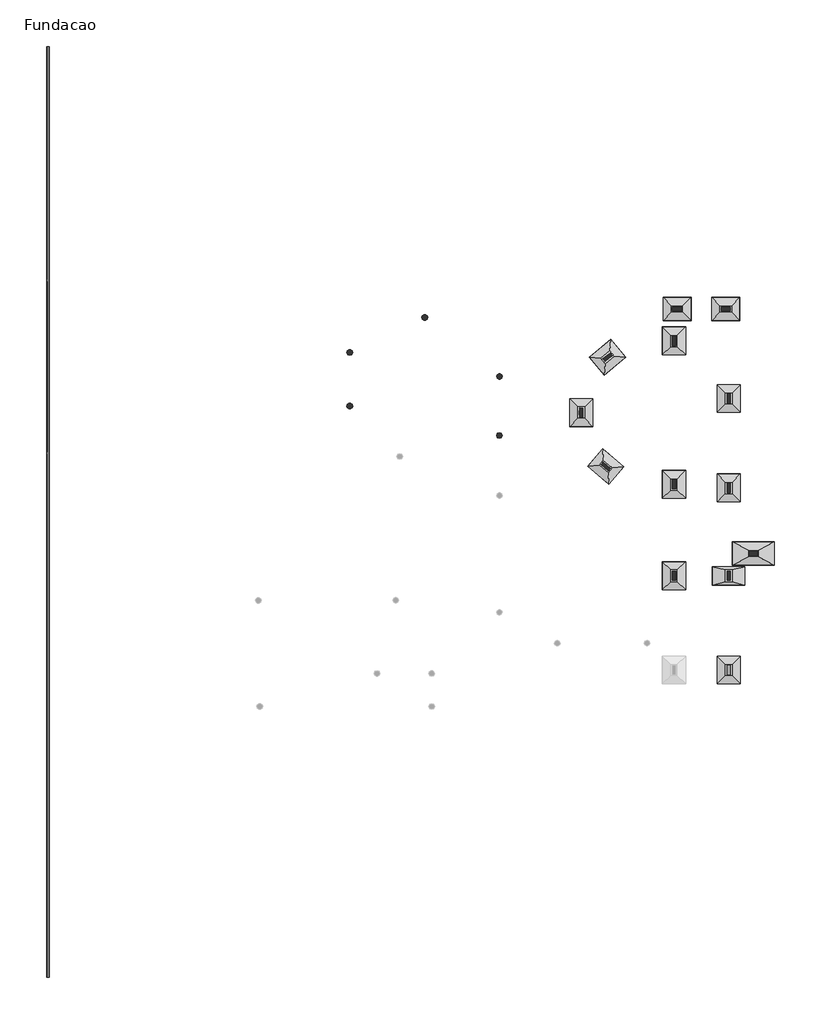
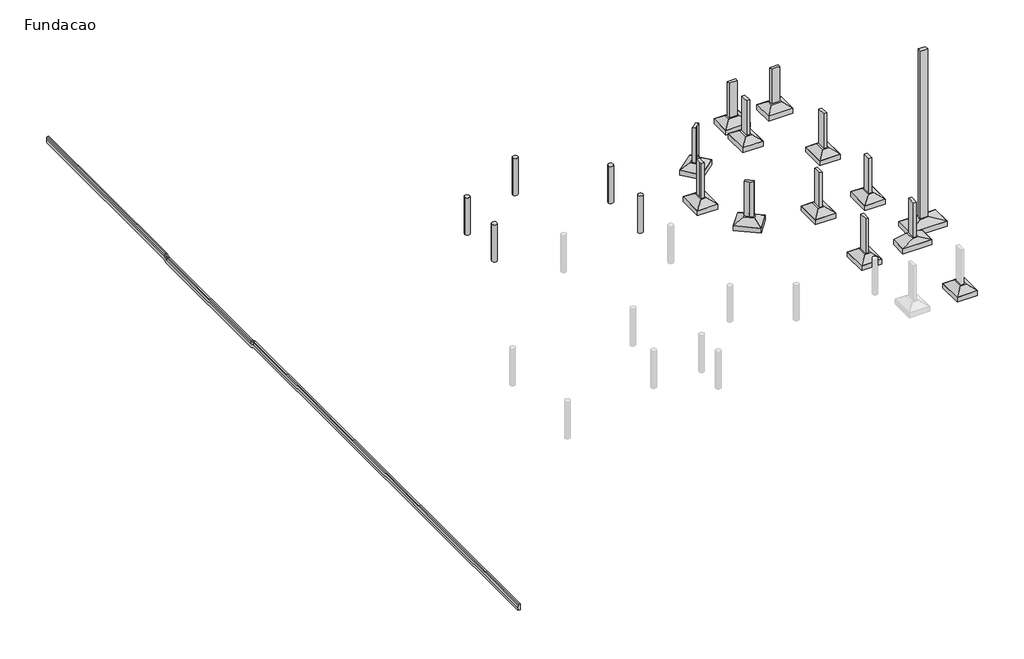
# One storey, part 2 of 2: 17 columns, 13 fasteners, 1 proxy.
"""IFC4 building model written with IfcOpenShell, lengths in millimetres."""

import ifcopenshell
import ifcopenshell.guid

model = None  # the IFC model being written
_history = None  # IfcOwnerHistory: only IFC2X3 demands one
_inside = {}  # id of a spatial element -> (the spatial element, [elements in it])
_under = {}  # id of a project, library or spatial element -> (it, [spatial elements below it])
_declared = {}  # id of a project -> (the project, [libraries it declares])
_typed = {}  # id of a type object -> (the type object, [elements of that type])
_made_of = {}  # id of a material, layer set ... -> (it, [elements and type objects made of it])


def new_model(schema):
    """Start an empty IFC model of exactly this schema.

    Asked for "IFC4X3", IfcOpenShell would pick the latest addendum, in which some entities
    have other attributes; the version numbers below select the first issue.
    IFC2X3 requires an IfcOwnerHistory on every rooted entity: one is made here for all.
    """
    global model, _history
    if schema == "IFC4X3":
        model = ifcopenshell.file(schema_version=(4, 3, 0, 0))
    else:
        model = ifcopenshell.file(schema=schema)
    _inside.clear()
    _under.clear()
    _declared.clear()
    _typed.clear()
    _made_of.clear()
    _history = None
    if model.schema == "IFC2X3":
        org = make("IfcOrganization", Name="unknown")
        user = make(
            "IfcPersonAndOrganization",
            ThePerson=make("IfcPerson", FamilyName="unknown"),
            TheOrganization=org,
        )
        app = make(
            "IfcApplication",
            ApplicationDeveloper=org,
            Version="unknown",
            ApplicationFullName="unknown",
            ApplicationIdentifier="unknown",
        )
        _history = make(
            "IfcOwnerHistory",
            OwningUser=user,
            OwningApplication=app,
            ChangeAction="ADDED",
            CreationDate=0,
        )
    return model


def make(cls, **values):
    """One entity of the class cls with the attributes given. An attribute that is None is left unset."""
    return model.create_entity(
        cls, **{name: value for name, value in values.items() if value is not None}
    )


def rooted(cls, **values):
    """An entity with a GlobalId (a new one), such as an element, a storey or a relation."""
    return make(cls, GlobalId=ifcopenshell.guid.new(), OwnerHistory=_history, **values)


def si_unit(unit_type, name, prefix=None):
    """IfcSIUnit, for example si_unit("LENGTHUNIT", "METRE", prefix="MILLI")."""
    return make("IfcSIUnit", UnitType=unit_type, Prefix=prefix, Name=name)


def assignment(units):
    """IfcUnitAssignment: the units of a project."""
    return None if units is None else make("IfcUnitAssignment", Units=units)


def point(xyz):
    """IfcCartesianPoint."""
    return None if xyz is None else make("IfcCartesianPoint", Coordinates=xyz)


def direction(xyz):
    """IfcDirection."""
    return None if xyz is None else make("IfcDirection", DirectionRatios=xyz)


def frame(location, z_axis=None, x_axis=None):
    """IfcAxis2Placement3D, a coordinate frame: its origin and axes. An axis left out is left unset."""
    return make(
        "IfcAxis2Placement3D",
        Location=point(location),
        Axis=direction(z_axis),
        RefDirection=direction(x_axis),
    )


def origin():
    """The frame at (0, 0, 0) with its axes left unset."""
    return frame((0.0, 0.0, 0.0))


def place(relative_to, where):
    """IfcLocalPlacement: puts the frame where relative to a parent placement (None: the world)."""
    return make(
        "IfcLocalPlacement", PlacementRelTo=relative_to, RelativePlacement=where
    )


def context(
    kind, dimensions, precision=None, world=None, true_north=None, identifier=None
):
    """IfcGeometricRepresentationContext, for example the 3D "Model" context."""
    return make(
        "IfcGeometricRepresentationContext",
        ContextIdentifier=identifier,
        ContextType=kind,
        CoordinateSpaceDimension=dimensions,
        Precision=precision,
        WorldCoordinateSystem=world,
        TrueNorth=true_north,
    )


def project(units=None, contexts=None):
    """IfcProject with its units and contexts."""
    return rooted(
        "IfcProject",
        Name="project",
        RepresentationContexts=contexts,
        UnitsInContext=assignment(units),
    )


def spatial(cls, under=None, at=None, **own):
    """A site, building, storey or space (cls), placed at a placement, below another one or the project."""
    s = rooted(cls, ObjectPlacement=at, **own)
    if under is not None:
        _under.setdefault(under.id(), (under, []))[1].append(s)
    return s


def polyline(points):
    """IfcPolyline through the points."""
    return make("IfcPolyline", Points=[point(p) for p in points])


def circle_curve(where, radius):
    """IfcCircle in the frame where."""
    return make("IfcCircle", Position=where, Radius=radius)


def ellipse_curve(where, semi_axis1, semi_axis2):
    """IfcEllipse in the frame where."""
    return make(
        "IfcEllipse", Position=where, SemiAxis1=semi_axis1, SemiAxis2=semi_axis2
    )


def outline(outer, holes=None, kind="AREA"):
    """IfcArbitraryClosedProfileDef: a profile drawn as a closed curve; with holes, ...WithVoids."""
    if holes is None:
        return make("IfcArbitraryClosedProfileDef", ProfileType=kind, OuterCurve=outer)
    return make(
        "IfcArbitraryProfileDefWithVoids",
        ProfileType=kind,
        OuterCurve=outer,
        InnerCurves=holes,
    )


def extrude(swept, where, along, depth):
    """IfcExtrudedAreaSolid: the profile swept, set in the frame where, extruded along a direction by depth."""
    return make(
        "IfcExtrudedAreaSolid",
        SweptArea=swept,
        Position=where,
        ExtrudedDirection=direction(along),
        Depth=depth,
    )


def faces_of(points, faces, orient=None, outer=None):
    """IfcFace entities. A face is a list of loops; a loop is a list of indices into points, from 0.

    orient and outer hold one flag for each loop. By default every Orientation is true, the
    first loop of a face is its IfcFaceOuterBound and the others are IfcFaceBound.
    """
    made = []
    for i, loops in enumerate(faces):
        bounds = []
        for j, loop in enumerate(loops):
            is_outer = j == 0 if outer is None else outer[i][j]
            bounds.append(
                make(
                    "IfcFaceOuterBound" if is_outer else "IfcFaceBound",
                    Bound=make("IfcPolyLoop", Polygon=[points[k] for k in loop]),
                    Orientation=True if orient is None else orient[i][j],
                )
            )
        made.append(make("IfcFace", Bounds=bounds))
    return made


def faceted_brep(points, faces, orient=None, outer=None, voids=None):
    """IfcFacetedBrep: a solid bounded by flat faces; with voids (closed shells), ...WithVoids."""
    shared = [point(p) for p in points]
    hull = make("IfcClosedShell", CfsFaces=faces_of(shared, faces, orient, outer))
    if voids is None:
        return make("IfcFacetedBrep", Outer=hull)
    return make(
        "IfcFacetedBrepWithVoids",
        Outer=hull,
        Voids=[
            make(cls, CfsFaces=faces_of(shared, fs, o, b)) for cls, fs, o, b in voids
        ],
    )


def shape(context_of_items, identifier, shape_type, items):
    """IfcShapeRepresentation: the items that make up one representation, for example the "Body"."""
    return make(
        "IfcShapeRepresentation",
        ContextOfItems=context_of_items,
        RepresentationIdentifier=identifier,
        RepresentationType=shape_type,
        Items=items,
    )


def source(mapping_origin, context_of_items, identifier, shape_type, items):
    """IfcRepresentationMap: a shape defined once, which mapped items show again and again."""
    return make(
        "IfcRepresentationMap",
        MappingOrigin=mapping_origin,
        MappedRepresentation=shape(context_of_items, identifier, shape_type, items),
    )


def transform(
    local_origin,
    x_axis=None,
    y_axis=None,
    z_axis=None,
    scale=None,
    scale2=None,
    scale3=None,
    uniform=True,
):
    """IfcCartesianTransformationOperator3D, or its non-uniform kind. x_axis, y_axis, z_axis: its Axis1, 2, 3."""
    if uniform:
        return make(
            "IfcCartesianTransformationOperator3D",
            Axis1=direction(x_axis),
            Axis2=direction(y_axis),
            LocalOrigin=point(local_origin),
            Scale=scale,
            Axis3=direction(z_axis),
        )
    return make(
        "IfcCartesianTransformationOperator3DnonUniform",
        Axis1=direction(x_axis),
        Axis2=direction(y_axis),
        LocalOrigin=point(local_origin),
        Scale=scale,
        Axis3=direction(z_axis),
        Scale2=scale2,
        Scale3=scale3,
    )


def mapped(mapping_source, mapping_target):
    """IfcMappedItem: shows the shape of a source again, moved by a transform."""
    return make(
        "IfcMappedItem", MappingSource=mapping_source, MappingTarget=mapping_target
    )


def made_of(thing, what):
    """Note that an element or type object is made of a material, layer set ...; save() writes the relation."""
    if what is not None:
        _made_of.setdefault(what.id(), (what, []))[1].append(thing)
    return thing


def element(
    cls,
    number,
    at=None,
    inside=None,
    cuts=None,
    type_object=None,
    material=None,
    context=None,
    identifier="Body",
    shape_type=None,
    held_by="IfcProductDefinitionShape",
    body=None,
    shapes=None,
    **own,
):
    """One element of the class cls, such as IfcWall. Its Tag is "e" and its number.

    at: its placement. inside: the storey or other place that contains it. cuts: it is an
    opening in that element (IfcRelVoidsElement). A single representation is given by context,
    identifier, shape_type and body (its items); several are given by shapes. held_by: the class
    of the entity that holds the representations. save() writes the other relations.
    """
    e = rooted(cls, Tag="e%d" % number, ObjectPlacement=at, **own)
    if body is not None:
        shapes = [shape(context, identifier, shape_type, body)]
    if shapes is not None:
        e.Representation = make(held_by, Representations=shapes)
    if inside is not None:
        _inside.setdefault(inside.id(), (inside, []))[1].append(e)
    if cuts is not None:
        rooted(
            "IfcRelVoidsElement", RelatingBuildingElement=cuts, RelatedOpeningElement=e
        )
    if type_object is not None:
        _typed.setdefault(type_object.id(), (type_object, []))[1].append(e)
    return made_of(e, material)


def aggregate(whole, parts):
    """IfcRelAggregates: a whole, such as a stair, and the parts it consists of."""
    return rooted("IfcRelAggregates", RelatingObject=whole, RelatedObjects=parts)


def save(model, path):
    """Write the relations noted so far, then the file.

    IfcRelAggregates (storeys below a building ...), IfcRelContainedInSpatialStructure (elements
    in a storey), IfcRelDefinesByType, IfcRelAssociatesMaterial and IfcRelDeclares: one each for
    every whole, place, type object, material and project.
    """
    for whole, parts in _under.values():
        aggregate(whole, parts)
    for where, things in _inside.values():
        rooted(
            "IfcRelContainedInSpatialStructure",
            RelatedElements=things,
            RelatingStructure=where,
        )
    for kind, things in _typed.values():
        rooted("IfcRelDefinesByType", RelatedObjects=things, RelatingType=kind)
    for what, things in _made_of.values():
        rooted("IfcRelAssociatesMaterial", RelatedObjects=things, RelatingMaterial=what)
    for by, libraries in _declared.values():
        rooted("IfcRelDeclares", RelatingContext=by, RelatedDefinitions=libraries)
    model.write(path)


def plane_surface(at):
    """IfcPlane: the flat surface through the origin of the frame at, square to its z axis."""
    return make("IfcPlane", Position=at)


def cylinder_surface(at, radius):
    """IfcCylindricalSurface: all points at the distance radius from the z axis of the frame at."""
    return make("IfcCylindricalSurface", Position=at, Radius=radius)


def advanced_brep(points, edges, surfaces, faces):
    """IfcAdvancedBrep: a solid bounded by faces that lie on surfaces and meet in shared edges.

    An edge is (start, end): straight between two places in points (the first is 0);
    or (start, end, curve); or (start, end, curve, False) where it runs against its curve.
    A face is (place in surfaces, loops), or (place, loops, False) where it looks against
    its surface's normal. A loop lists edges by number (the first is 1), with a minus sign
    where the edge is run from its end to its start. The first loop is the outer one.
    """
    corners = [point(p) for p in points]
    vertices = [make("IfcVertexPoint", VertexGeometry=c) for c in corners]
    made = []
    for start, end, *more in edges:
        made.append(
            make(
                "IfcEdgeCurve",
                EdgeStart=vertices[start],
                EdgeEnd=vertices[end],
                EdgeGeometry=more[0] if more else make("IfcPolyline", Points=[corners[start], corners[end]]),
                SameSense=more[1] if len(more) > 1 else True,
            )
        )
    hull = []
    for where, loops, *sense in faces:
        bounds = []
        for j, loop in enumerate(loops):
            ring = [make("IfcOrientedEdge", EdgeElement=made[abs(k) - 1], Orientation=k > 0) for k in loop]
            bounds.append(
                make(
                    "IfcFaceOuterBound" if j == 0 else "IfcFaceBound",
                    Bound=make("IfcEdgeLoop", EdgeList=ring),
                    Orientation=True,
                )
            )
        hull.append(make("IfcAdvancedFace", Bounds=bounds, FaceSurface=surfaces[where], SameSense=sense[0] if sense else True))
    return make("IfcAdvancedBrep", Outer=make("IfcClosedShell", CfsFaces=hull))


def meio_fio_meio_fio_c5939b1e(model_context):
    return source(origin(), model_context, "Body", "AdvancedBrep", [
        advanced_brep(
        [(-19460.281307, 17327.5225294, 100.0), (-19460.281307, 17327.5225294, -200.0), (-19580.281307, 17327.5225294, -200.0), (-19580.281307, 17327.5225294, -50.0), (-19560.334366, 17327.5225294, 74.7371665), (-19530.7107394, 17327.5225294, 100.0), (-19460.281307, 7304.4300153, 100.0), (-19460.281307, 7104.4300153, 20.0), (-19460.281307, 4.4300153, 20.0), (-19460.281307, -195.5699847, 100.0), (-19460.281307, -22700.938406, 100.0), (-19460.281307, -22700.938406, -200.0), (-19460.281307, -253.3447058, -200.0), (-19460.281307, -53.3447058, -280.0), (-19460.281307, 7162.2047364, -280.0), (-19460.281307, 7362.2047364, -200.0), (-19580.281307, 7362.2047364, -200.0), (-19580.281307, 7162.2047364, -280.0), (-19580.281307, -53.3447058, -280.0), (-19580.281307, -253.3447058, -200.0), (-19580.281307, -22700.938406, -200.0), (-19580.281307, -22700.938406, -50.0), (-19580.281307, -224.4573452, -50.0), (-19580.281307, -24.4573452, -130.0), (-19580.281307, 7133.3173758, -130.0), (-19580.281307, 7333.3173758, -50.0), (-19560.334366, 7309.2951925, 74.7371665), (-19530.7107394, 7304.4300153, 100.0), (-19560.334366, 7109.2951925, -5.2628335), (-19530.7107394, 7104.4300153, 20.0), (-19560.334366, -0.4351619, -5.2628335), (-19530.7107394, 4.4300153, 20.0), (-19560.334366, -200.4351619, 74.7371665), (-19530.7107394, -195.5699847, 100.0), (-19530.7107394, -22700.938406, 100.0), (-19560.334366, -22700.938406, 74.7371665)],
        [
            (0, 1),
            (1, 2),
            (2, 3),
            (3, 4),
            (4, 5, circle_curve(frame((-19530.7107394, 17327.5225294, 70.0), z_axis=(0.0, 1.0, 0.0), x_axis=(-1.0, 0.0, 0.0)), 30.0)),
            (5, 0),
            (0, 6),
            (6, 7),
            (7, 8),
            (8, 9),
            (9, 10),
            (10, 11),
            (11, 12),
            (12, 13),
            (13, 14),
            (14, 15),
            (15, 1),
            (15, 16),
            (16, 2),
            (16, 17),
            (17, 18),
            (18, 19),
            (19, 20),
            (20, 21),
            (21, 22),
            (22, 23),
            (23, 24),
            (24, 25),
            (25, 3),
            (25, 26),
            (26, 4),
            (26, 27, ellipse_curve(frame((-19530.7107394, 7310.2074874, 70.0), z_axis=(0.0, 0.9819563867314226, 0.18910752115494767), x_axis=(0.0, 0.18910752115494667, -0.9819563867314226)), 30.551255, 30.0)),
            (27, 5),
            (27, 6),
            (14, 17),
            (24, 28),
            (28, 26),
            (28, 29, ellipse_curve(frame((-19530.7107394, 7110.2074874, -10.0), z_axis=(0.0, 0.9819563867314226, 0.18910752115494764), x_axis=(0.0, -0.18910752115494842, 0.9819563867314223)), 30.551255, 30.0)),
            (29, 27),
            (29, 7),
            (13, 18),
            (23, 30),
            (30, 28),
            (30, 31, ellipse_curve(frame((-19530.7107394, -1.3474568, -10.0), z_axis=(0.0, 0.9819563867314217, -0.1891075211549513), x_axis=(0.0, 0.18910752115495252, 0.9819563867314217)), 30.551255, 30.0)),
            (31, 29),
            (31, 8),
            (12, 19),
            (22, 32),
            (32, 30),
            (32, 33, ellipse_curve(frame((-19530.7107394, -201.3474568, 70.0), z_axis=(0.0, 0.9819563867314217, -0.18910752115495139), x_axis=(0.0, -0.18910752115495078, -0.9819563867314218)), 30.551255, 30.0)),
            (33, 31),
            (33, 9),
            (10, 34),
            (34, 35, circle_curve(frame((-19530.7107394, -22700.938406, 70.0), z_axis=(0.0, -1.0, 0.0), x_axis=(-1.0, 0.0, 0.0)), 30.0)),
            (35, 21),
            (20, 11),
            (35, 32),
            (34, 33),
        ],
        [
            plane_surface(frame((-19460.281307, 17327.5225294, 100.0), z_axis=(0.0, 1.0, 0.0), x_axis=(0.0, 0.0, 1.0))),
            plane_surface(frame((-19460.281307, 17327.5225294, 100.0), z_axis=(1.0, 0.0, 0.0), x_axis=(0.0, -1.0, 0.0))),
            plane_surface(frame((-19460.281307, 17327.5225294, -200.0), z_axis=(0.0, 0.0, -1.0), x_axis=(0.0, -1.0, 0.0))),
            plane_surface(frame((-19580.281307, 17327.5225294, -200.0), z_axis=(-1.0, 0.0, 0.0), x_axis=(0.0, -1.0, 0.0))),
            plane_surface(frame((-19580.281307, 17327.5225294, -50.0), z_axis=(-0.9874542202157147, 0.0, 0.15790555081495689), x_axis=(0.0, -1.0, 0.0))),
            cylinder_surface(frame((-19530.7107394, 17327.5225294, 70.0), z_axis=(0.0, 1.0, 0.0), x_axis=(-1.0, 0.0, 0.0)), 30.0),
            plane_surface(frame((-19530.7107394, 17327.5225294, 100.0), z_axis=(0.0, 0.0, 1.0), x_axis=(0.0, -1.0, 0.0))),
            plane_surface(frame((-19460.281307, 7362.2047364, -200.0), z_axis=(0.0, 0.3713906763540969, -0.9284766908852621), x_axis=(0.0, -0.9284766908852621, -0.3713906763540969))),
            plane_surface(frame((-19580.281307, 7333.3173758, -50.0), z_axis=(-0.9874542202157147, -0.05864464931723302, 0.1466116232930858), x_axis=(0.0, -0.9284766908852622, -0.3713906763540966))),
            cylinder_surface(frame((-19530.7107394, 7315.5717356, 72.1456993), z_axis=(0.0, 0.9284766908852621, 0.3713906763540969), x_axis=(-1.0, 0.0, 0.0)), 30.0),
            plane_surface(frame((-19530.7107394, 7304.4300153, 100.0), z_axis=(0.0, -0.37139067635409667, 0.9284766908852622), x_axis=(0.0, -0.9284766908852622, -0.37139067635409667))),
            plane_surface(frame((-19460.281307, 7162.2047364, -280.0), z_axis=(0.0, 0.0, -1.0), x_axis=(0.0, -1.0, 0.0))),
            plane_surface(frame((-19580.281307, 7133.3173758, -130.0), z_axis=(-0.9874542202157146, 0.0, 0.15790555081495686), x_axis=(0.0, -1.0, 0.0))),
            cylinder_surface(frame((-19530.7107394, 7104.4300153, -10.0), z_axis=(0.0, 1.0, 0.0), x_axis=(-1.0, 0.0, 0.0)), 30.0),
            plane_surface(frame((-19530.7107394, 7104.4300153, 20.0), z_axis=(0.0, 0.0, 1.0), x_axis=(0.0, -1.0, 0.0))),
            plane_surface(frame((-19460.281307, -53.3447058, -280.0), z_axis=(0.0, -0.37139067635410367, -0.9284766908852594), x_axis=(0.0, -0.9284766908852594, 0.37139067635410367))),
            plane_surface(frame((-19580.281307, -24.4573452, -130.0), z_axis=(-0.9874542202157147, 0.05864464931723411, 0.14661162329308536), x_axis=(0.0, -0.9284766908852594, 0.37139067635410355))),
            cylinder_surface(frame((-19530.7107394, -6.711705, -7.8543007), z_axis=(0.0, 0.9284766908852593, -0.3713906763541038), x_axis=(-1.0, 0.0, 0.0)), 30.0),
            plane_surface(frame((-19530.7107394, 4.4300153, 20.0), z_axis=(0.0, 0.3713906763541038, 0.9284766908852593), x_axis=(0.0, -0.9284766908852593, 0.3713906763541038))),
            plane_surface(frame((-19460.281307, -22700.938406, 100.0), z_axis=(0.0, -1.0, 0.0), x_axis=(0.0, 0.0, 1.0))),
            plane_surface(frame((-19460.281307, -253.3447058, -200.0), z_axis=(0.0, 0.0, -1.0), x_axis=(0.0, -1.0, 0.0))),
            plane_surface(frame((-19580.281307, -224.4573452, -50.0), z_axis=(-0.9874542202157146, 0.0, 0.15790555081495683), x_axis=(0.0, -1.0, 0.0))),
            cylinder_surface(frame((-19530.7107394, -195.5699847, 70.0), z_axis=(0.0, 1.0, 0.0), x_axis=(-1.0, 0.0, 0.0)), 30.0),
            plane_surface(frame((-19530.7107394, -195.5699847, 100.0), z_axis=(0.0, 0.0, 1.0), x_axis=(0.0, -1.0, 0.0))),
        ],
        [
            (0, [[1, 2, 3, 4, 5, 6]]),
            (1, [[-1, 7, 8, 9, 10, 11, 12, 13, 14, 15, 16, 17]]),
            (2, [[-2, -17, 18, 19]]),
            (3, [[-3, -19, 20, 21, 22, 23, 24, 25, 26, 27, 28, 29]]),
            (4, [[-4, -29, 30, 31]]),
            (5, [[-5, -31, 32, 33]]),
            (6, [[-6, -33, 34, -7]]),
            (7, [[-18, -16, 35, -20]]),
            (8, [[-30, -28, 36, 37]]),
            (9, [[-32, -37, 38, 39]]),
            (10, [[-34, -39, 40, -8]]),
            (11, [[-35, -15, 41, -21]]),
            (12, [[-36, -27, 42, 43]]),
            (13, [[-38, -43, 44, 45]]),
            (14, [[-40, -45, 46, -9]]),
            (15, [[-41, -14, 47, -22]]),
            (16, [[-42, -26, 48, 49]]),
            (17, [[-44, -49, 50, 51]]),
            (18, [[-46, -51, 52, -10]]),
            (19, [[53, 54, 55, -24, 56, -12]]),
            (20, [[-47, -13, -56, -23]]),
            (21, [[-48, -25, -55, 57]]),
            (22, [[-50, -57, -54, 58]]),
            (23, [[-52, -58, -53, -11]]),
        ],
    ),
    ])


def s14_8166d2be(model_context):
    return source(origin(), model_context, "Body", "SolidModel", [
        faceted_brep([(-55.0, 0.0, 0.0), (-345.0, 0.0, 0.0), (-345.0, -400.0, 0.0), (-55.0, -400.0, 0.0), (300.0, 700.0, -250.0), (300.0, -1100.0, -250.0), (-700.0, -1100.0, -250.0), (-700.0, 700.0, -250.0)], [[[0, 1, 2, 3]], [[4, 5, 6, 7]], [[4, 7, 1, 0]], [[7, 6, 2, 1]], [[6, 5, 3, 2]], [[5, 4, 0, 3]]]),
        extrude(outline(polyline([(300.0, 700.0), (300.0, -1100.0), (-700.0, -1100.0), (-700.0, 700.0), (300.0, 700.0)])), frame((0.0, 0.0, -500.0), z_axis=(0.0, 0.0, 1.0), x_axis=(1.0, 0.0, 0.0)), (0.0, 0.0, 1.0), 250.0),
    ])


def sps1_6b3be553(model_context):
    return source(origin(), model_context, "Body", "SolidModel", [
        faceted_brep([(-55.0, 50.0, 0.0), (-345.0, 50.0, 0.0), (-345.0, -450.0, 0.0), (-55.0, -450.0, 0.0), (300.0, 400.0, -250.0), (300.0, -800.0, -250.0), (-700.0, -800.0, -250.0), (-700.0, 400.0, -250.0)], [[[0, 1, 2, 3]], [[4, 5, 6, 7]], [[4, 7, 1, 0]], [[7, 6, 2, 1]], [[6, 5, 3, 2]], [[5, 4, 0, 3]]]),
        extrude(outline(polyline([(300.0, 400.0), (300.0, -800.0), (-700.0, -800.0), (-700.0, 400.0), (300.0, 400.0)])), frame((0.0, 0.0, -500.0), z_axis=(0.0, 0.0, 1.0), x_axis=(1.0, 0.0, 0.0)), (0.0, 0.0, 1.0), 250.0),
    ])


def sps11_3ae28187(model_context):
    return source(origin(), model_context, "Body", "SolidModel", [
        faceted_brep([(-55.0, 50.0, 0.0), (-345.0, 50.0, 0.0), (-345.0, -450.0, 0.0), (-55.0, -450.0, 0.0), (500.0, 200.0, -250.0), (500.0, -600.0, -250.0), (-900.0, -600.0, -250.0), (-900.0, 200.0, -250.0)], [[[0, 1, 2, 3]], [[4, 5, 6, 7]], [[4, 7, 1, 0]], [[7, 6, 2, 1]], [[6, 5, 3, 2]], [[5, 4, 0, 3]]]),
        extrude(outline(polyline([(500.0, 200.0), (500.0, -600.0), (-900.0, -600.0), (-900.0, 200.0), (500.0, 200.0)])), frame((0.0, 0.0, -500.0), z_axis=(0.0, 0.0, 1.0), x_axis=(1.0, 0.0, 0.0)), (0.0, 0.0, 1.0), 250.0),
    ])


model = new_model("IFC4")

# Units and contexts
model_context = context("Model", 3, world=origin())
ifc_project = project(units=[si_unit("LENGTHUNIT", "METRE", prefix="MILLI")], contexts=[model_context])

# Site, building, storey
site = spatial("IfcSite", under=ifc_project)
building = spatial("IfcBuilding", under=site)
storey = spatial("IfcBuildingStorey", under=building, Name="Fundacao", Elevation=-1200.0)

# Proxy
placement = place(None, origin())
meio_fio_meio_fio_shape = meio_fio_meio_fio_c5939b1e(model_context)
element("IfcBuildingElementProxy", 1, Name="MEIO-FIO : MEIO-FIO", ObjectType="MEIO-FIO : MEIO-FIO", at=placement, inside=storey, context=model_context, shape_type="MappedRepresentation", body=[
    mapped(meio_fio_meio_fio_shape, transform((0.0, 0.0, 0.0), x_axis=(1.0, 0.0, 0.0), y_axis=(0.0, 1.0, 0.0), z_axis=(0.0, 0.0, 1.0))),
])

# Columns
element("IfcColumn", 2, ObjectType="TQS - Pilar circular : TQS - Pilar circular 25.0cm", at=placement, inside=storey, context=model_context, shape_type="AdvancedBrep", body=[
    advanced_brep(
    [(-3446.281307, 5679.4300153, -1500.0), (-3196.281307, 5679.4300153, -1500.0), (-3446.281307, 5679.4300153, 430.0), (-3402.499945, 5774.4486073, 430.0), (-3240.0409229, 5774.4300153, 430.0), (-3196.281307, 5679.4300153, 430.0), (-3240.0409229, 5584.4300153, 430.0), (-3402.499945, 5584.4114233, 430.0)],
    [
        (0, 1, circle_curve(frame((-3321.281307, 5679.4300153, -1500.0), z_axis=(0.0, 0.0, -1.0), x_axis=(1.0, 0.0, 0.0)), 125.0)),
        (1, 0, circle_curve(frame((-3321.281307, 5679.4300153, -1500.0), z_axis=(0.0, 0.0, -1.0), x_axis=(1.0, 0.0, 0.0)), 125.0)),
        (2, 3, circle_curve(frame((-3321.281307, 5679.4300153, 430.0), z_axis=(0.0, 0.0, -1.0), x_axis=(1.0, 0.0, 0.0)), 125.0)),
        (3, 4, circle_curve(frame((-3321.281307, 5679.4300153, 430.0), z_axis=(0.0, 0.0, -1.0), x_axis=(1.0, 0.0, 0.0)), 125.0)),
        (4, 5, circle_curve(frame((-3321.281307, 5679.4300153, 430.0), z_axis=(0.0, 0.0, -1.0), x_axis=(1.0, 0.0, 0.0)), 125.0)),
        (5, 1),
        (0, 2),
        (5, 6, circle_curve(frame((-3321.281307, 5679.4300153, 430.0), z_axis=(0.0, 0.0, -1.0), x_axis=(1.0, 0.0, 0.0)), 125.0)),
        (6, 7, circle_curve(frame((-3321.281307, 5679.4300153, 430.0), z_axis=(0.0, 0.0, -1.0), x_axis=(1.0, 0.0, 0.0)), 125.0)),
        (7, 2, circle_curve(frame((-3321.281307, 5679.4300153, 430.0), z_axis=(0.0, 0.0, -1.0), x_axis=(1.0, 0.0, 0.0)), 125.0)),
    ],
    [
        plane_surface(frame((-3196.281307, 5679.4300153, -1500.0), z_axis=(0.0, 0.0, -1.0), x_axis=(0.0, -1.0, 0.0))),
        cylinder_surface(frame((-3321.281307, 5679.4300153, -1500.0), z_axis=(0.0, 0.0, 1.0), x_axis=(1.0, 0.0, 0.0)), 125.0),
        plane_surface(frame((-3196.281307, 5679.4300153, 430.0), z_axis=(0.0, 0.0, 1.0), x_axis=(0.0, 1.0, 0.0))),
    ],
    [
        (0, [[1, 2]]),
        (1, [[3, 4, 5, 6, -1, 7]]),
        (1, [[8, 9, 10, -7, -2, -6]]),
        (2, [[-10, -9, -8, -5, -4, -3]]),
    ],
),
])
element("IfcColumn", 3, ObjectType="TQS - Pilar circular : TQS - Pilar circular 25.0cm", at=placement, inside=storey, context=model_context, shape_type="AdvancedBrep", body=[
    advanced_brep(
    [(-232.281307, 604.4300152, -1500.0), (17.718693, 604.4300152, -1500.0), (-232.281307, 604.4300152, 430.0), (-202.281307, 685.6703993, 430.0), (-12.281307, 685.6703993, 430.0), (17.718693, 604.4300152, 430.0), (-12.281307, 523.1896312, 430.0), (-202.281307, 523.1896312, 430.0)],
    [
        (0, 1, circle_curve(frame((-107.281307, 604.4300152, -1500.0), z_axis=(0.0, 0.0, -1.0), x_axis=(1.0, 0.0, 0.0)), 125.0)),
        (1, 0, circle_curve(frame((-107.281307, 604.4300152, -1500.0), z_axis=(0.0, 0.0, -1.0), x_axis=(1.0, 0.0, 0.0)), 125.0)),
        (2, 3, circle_curve(frame((-107.281307, 604.4300152, 430.0), z_axis=(0.0, 0.0, -1.0), x_axis=(1.0, 0.0, 0.0)), 125.0)),
        (3, 4, circle_curve(frame((-107.281307, 604.4300152, 430.0), z_axis=(0.0, 0.0, -1.0), x_axis=(1.0, 0.0, 0.0)), 125.0)),
        (4, 5, circle_curve(frame((-107.281307, 604.4300152, 430.0), z_axis=(0.0, 0.0, -1.0), x_axis=(1.0, 0.0, 0.0)), 125.0)),
        (5, 1),
        (0, 2),
        (5, 6, circle_curve(frame((-107.281307, 604.4300152, 430.0), z_axis=(0.0, 0.0, -1.0), x_axis=(1.0, 0.0, 0.0)), 125.0)),
        (6, 7, circle_curve(frame((-107.281307, 604.4300152, 430.0), z_axis=(0.0, 0.0, -1.0), x_axis=(1.0, 0.0, 0.0)), 125.0)),
        (7, 2, circle_curve(frame((-107.281307, 604.4300152, 430.0), z_axis=(0.0, 0.0, -1.0), x_axis=(1.0, 0.0, 0.0)), 125.0)),
    ],
    [
        plane_surface(frame((17.718693, 604.4300152, -1500.0), z_axis=(0.0, 0.0, -1.0), x_axis=(0.0, -1.0, 0.0))),
        cylinder_surface(frame((-107.281307, 604.4300152, -1500.0), z_axis=(0.0, 0.0, 1.0), x_axis=(1.0, 0.0, 0.0)), 125.0),
        plane_surface(frame((17.718693, 604.4300152, 430.0), z_axis=(0.0, 0.0, 1.0), x_axis=(0.0, 1.0, 0.0))),
    ],
    [
        (0, [[1, 2]]),
        (1, [[3, 4, 5, 6, -1, 7]]),
        (1, [[8, 9, 10, -7, -2, -6]]),
        (2, [[-10, -9, -8, -5, -4, -3]]),
    ],
),
])
element("IfcColumn", 4, ObjectType="TQS - Pilar circular : TQS - Pilar circular 25.0cm", at=placement, inside=storey, context=model_context, shape_type="AdvancedBrep", body=[
    advanced_brep(
    [(-232.281307, 3141.9300152, -1500.0), (17.718693, 3141.9300152, -1500.0), (-232.281307, 3141.9300152, 430.0), (-202.281307, 3223.1703993, 430.0), (-12.281307, 3223.1703993, 430.0), (17.718693, 3141.9300152, 430.0), (-12.281307, 3060.6896312, 430.0), (-202.281307, 3060.6896312, 430.0)],
    [
        (0, 1, circle_curve(frame((-107.281307, 3141.9300152, -1500.0), z_axis=(0.0, 0.0, -1.0), x_axis=(1.0, 0.0, 0.0)), 125.0)),
        (1, 0, circle_curve(frame((-107.281307, 3141.9300152, -1500.0), z_axis=(0.0, 0.0, -1.0), x_axis=(1.0, 0.0, 0.0)), 125.0)),
        (2, 3, circle_curve(frame((-107.281307, 3141.9300152, 430.0), z_axis=(0.0, 0.0, -1.0), x_axis=(1.0, 0.0, 0.0)), 125.0)),
        (3, 4, circle_curve(frame((-107.281307, 3141.9300152, 430.0), z_axis=(0.0, 0.0, -1.0), x_axis=(1.0, 0.0, 0.0)), 125.0)),
        (4, 5, circle_curve(frame((-107.281307, 3141.9300152, 430.0), z_axis=(0.0, 0.0, -1.0), x_axis=(1.0, 0.0, 0.0)), 125.0)),
        (5, 1),
        (0, 2),
        (5, 6, circle_curve(frame((-107.281307, 3141.9300152, 430.0), z_axis=(0.0, 0.0, -1.0), x_axis=(1.0, 0.0, 0.0)), 125.0)),
        (6, 7, circle_curve(frame((-107.281307, 3141.9300152, 430.0), z_axis=(0.0, 0.0, -1.0), x_axis=(1.0, 0.0, 0.0)), 125.0)),
        (7, 2, circle_curve(frame((-107.281307, 3141.9300152, 430.0), z_axis=(0.0, 0.0, -1.0), x_axis=(1.0, 0.0, 0.0)), 125.0)),
    ],
    [
        plane_surface(frame((17.718693, 3141.9300152, -1500.0), z_axis=(0.0, 0.0, -1.0), x_axis=(0.0, -1.0, 0.0))),
        cylinder_surface(frame((-107.281307, 3141.9300152, -1500.0), z_axis=(0.0, 0.0, 1.0), x_axis=(1.0, 0.0, 0.0)), 125.0),
        plane_surface(frame((17.718693, 3141.9300152, 430.0), z_axis=(0.0, 0.0, 1.0), x_axis=(0.0, 1.0, 0.0))),
    ],
    [
        (0, [[1, 2]]),
        (1, [[3, 4, 5, 6, -1, 7]]),
        (1, [[8, 9, 10, -7, -2, -6]]),
        (2, [[-10, -9, -8, -5, -4, -3]]),
    ],
),
])
element("IfcColumn", 5, ObjectType="TQS - Pilar circular : TQS - Pilar circular 25.0cm", at=placement, inside=storey, context=model_context, shape_type="AdvancedBrep", body=[
    advanced_brep(
    [(-6671.281307, 4171.2050153, -1500.0), (-6421.281307, 4171.2050153, -1500.0), (-6671.281307, 4171.2050153, 430.0), (-6630.281307, 4263.7739086, 430.0), (-6440.281307, 4237.4545436, 430.0), (-6421.281307, 4171.2050153, 430.0), (-6440.281307, 4104.955487, 430.0), (-6630.281307, 4078.636122, 430.0)],
    [
        (0, 1, circle_curve(frame((-6546.281307, 4171.2050153, -1500.0), z_axis=(0.0, 0.0, -1.0), x_axis=(1.0, 0.0, 0.0)), 125.0)),
        (1, 0, circle_curve(frame((-6546.281307, 4171.2050153, -1500.0), z_axis=(0.0, 0.0, -1.0), x_axis=(1.0, 0.0, 0.0)), 125.0)),
        (2, 3, circle_curve(frame((-6546.281307, 4171.2050153, 430.0), z_axis=(0.0, 0.0, -1.0), x_axis=(1.0, 0.0, 0.0)), 125.0)),
        (3, 4, circle_curve(frame((-6546.281307, 4171.2050153, 430.0), z_axis=(0.0, 0.0, -1.0), x_axis=(1.0, 0.0, 0.0)), 125.0)),
        (4, 5, circle_curve(frame((-6546.281307, 4171.2050153, 430.0), z_axis=(0.0, 0.0, -1.0), x_axis=(1.0, 0.0, 0.0)), 125.0)),
        (5, 1),
        (0, 2),
        (5, 6, circle_curve(frame((-6546.281307, 4171.2050153, 430.0), z_axis=(0.0, 0.0, -1.0), x_axis=(1.0, 0.0, 0.0)), 125.0)),
        (6, 7, circle_curve(frame((-6546.281307, 4171.2050153, 430.0), z_axis=(0.0, 0.0, -1.0), x_axis=(1.0, 0.0, 0.0)), 125.0)),
        (7, 2, circle_curve(frame((-6546.281307, 4171.2050153, 430.0), z_axis=(0.0, 0.0, -1.0), x_axis=(1.0, 0.0, 0.0)), 125.0)),
    ],
    [
        plane_surface(frame((-6421.281307, 4171.2050153, -1500.0), z_axis=(0.0, 0.0, -1.0), x_axis=(0.0, -1.0, 0.0))),
        cylinder_surface(frame((-6546.281307, 4171.2050153, -1500.0), z_axis=(0.0, 0.0, 1.0), x_axis=(1.0, 0.0, 0.0)), 125.0),
        plane_surface(frame((-6421.281307, 4171.2050153, 430.0), z_axis=(0.0, 0.0, 1.0), x_axis=(0.0, 1.0, 0.0))),
    ],
    [
        (0, [[1, 2]]),
        (1, [[3, 4, 5, 6, -1, 7]]),
        (1, [[8, 9, 10, -7, -2, -6]]),
        (2, [[-10, -9, -8, -5, -4, -3]]),
    ],
),
])
element("IfcColumn", 6, ObjectType="TQS - Pilar circular : TQS - Pilar circular 25.0cm", at=placement, inside=storey, context=model_context, shape_type="AdvancedBrep", body=[
    advanced_brep(
    [(-6666.2813069, 1866.7050153, -1500.0), (-6416.2813069, 1866.7050153, -1500.0), (-6666.2813069, 1866.7050153, 430.0), (-6630.281307, 1954.4774483, 430.0), (-6440.281307, 1940.3528259, 430.0), (-6416.2813069, 1866.7050153, 430.0), (-6440.281307, 1793.0572047, 430.0), (-6630.281307, 1778.9325823, 430.0)],
    [
        (0, 1, circle_curve(frame((-6541.2813069, 1866.7050153, -1500.0), z_axis=(0.0, 0.0, -1.0), x_axis=(1.0, 0.0, 0.0)), 125.0)),
        (1, 0, circle_curve(frame((-6541.2813069, 1866.7050153, -1500.0), z_axis=(0.0, 0.0, -1.0), x_axis=(1.0, 0.0, 0.0)), 125.0)),
        (2, 3, circle_curve(frame((-6541.2813069, 1866.7050153, 430.0), z_axis=(0.0, 0.0, -1.0), x_axis=(1.0, 0.0, 0.0)), 125.0)),
        (3, 4, circle_curve(frame((-6541.2813069, 1866.7050153, 430.0), z_axis=(0.0, 0.0, -1.0), x_axis=(1.0, 0.0, 0.0)), 125.0)),
        (4, 5, circle_curve(frame((-6541.2813069, 1866.7050153, 430.0), z_axis=(0.0, 0.0, -1.0), x_axis=(1.0, 0.0, 0.0)), 125.0)),
        (5, 1),
        (0, 2),
        (5, 6, circle_curve(frame((-6541.2813069, 1866.7050153, 430.0), z_axis=(0.0, 0.0, -1.0), x_axis=(1.0, 0.0, 0.0)), 125.0)),
        (6, 7, circle_curve(frame((-6541.2813069, 1866.7050153, 430.0), z_axis=(0.0, 0.0, -1.0), x_axis=(1.0, 0.0, 0.0)), 125.0)),
        (7, 2, circle_curve(frame((-6541.2813069, 1866.7050153, 430.0), z_axis=(0.0, 0.0, -1.0), x_axis=(1.0, 0.0, 0.0)), 125.0)),
    ],
    [
        plane_surface(frame((-6416.2813069, 1866.7050153, -1500.0), z_axis=(0.0, 0.0, -1.0), x_axis=(0.0, -1.0, 0.0))),
        cylinder_surface(frame((-6541.2813069, 1866.7050153, -1500.0), z_axis=(0.0, 0.0, 1.0), x_axis=(1.0, 0.0, 0.0)), 125.0),
        plane_surface(frame((-6416.2813069, 1866.7050153, 430.0), z_axis=(0.0, 0.0, 1.0), x_axis=(0.0, 1.0, 0.0))),
    ],
    [
        (0, [[1, 2]]),
        (1, [[3, 4, 5, 6, -1, 7]]),
        (1, [[8, 9, 10, -7, -2, -6]]),
        (2, [[-10, -9, -8, -5, -4, -3]]),
    ],
),
])
element("IfcColumn", 7, ObjectType="TQS - Pilar retangular : 14.0 x 40.0", at=placement, inside=storey, context=model_context, shape_type="Brep", body=[
    faceted_brep([(9822.718693, 5969.4300153, -1450.0), (9682.718693, 5969.4300153, -1450.0), (9422.718693, 5969.4300153, -1450.0), (9422.718693, 6109.4300153, -1450.0), (9822.718693, 6109.4300153, -1450.0), (9822.718693, 5969.4300153, 350.0), (9682.718693, 5969.4300153, 350.0), (9422.718693, 5969.4300153, 350.0), (9422.718693, 6109.4300153, 350.0), (9822.718693, 6109.4300153, 350.0)], [[[0, 1, 2, 3, 4]], [[5, 6, 7, 2, 1, 0]], [[7, 8, 3, 2]], [[8, 9, 4, 3]], [[9, 5, 0, 4]], [[5, 9, 8, 7, 6]]]),
])
element("IfcColumn", 8, ObjectType="TQS - Pilar retangular : 14.0 x 40.0", at=placement, inside=storey, context=model_context, shape_type="Brep", body=[
    faceted_brep([(7734.718693, 5969.4300153, -1450.0), (7474.7218272, 5969.4300153, -1450.0), (7334.718693, 5969.4300153, -1450.0), (7334.718693, 6109.4300153, -1450.0), (7734.718693, 6109.4300153, -1450.0), (7734.718693, 5969.4300153, 350.0), (7474.7218272, 5969.4300153, 350.0), (7334.718693, 5969.4300153, 350.0), (7334.718693, 6109.4300153, 350.0), (7734.718693, 6109.4300153, 350.0)], [[[0, 1, 2, 3, 4]], [[5, 6, 7, 2, 1, 0]], [[7, 8, 3, 2]], [[8, 9, 4, 3]], [[9, 5, 0, 4]], [[5, 9, 8, 7, 6]]]),
])
element("IfcColumn", 9, ObjectType="TQS - Pilar retangular : 14.0 x 40.0", at=placement, inside=storey, context=model_context, shape_type="Brep", body=[
    faceted_brep([(7334.7218272, 4470.7003679, -1450.0), (7334.7218272, 4614.8968948, -1450.0), (7334.7218272, 4870.7003679, -1450.0), (7474.7218272, 4870.7003679, -1450.0), (7474.7218272, 4470.7003679, -1450.0), (7334.7218272, 4470.7003679, -1250.0), (7334.7218272, 4470.7003679, 350.0), (7334.7218272, 4614.8968948, 350.0), (7334.7218272, 4870.7003679, 350.0), (7474.7218272, 4870.7003679, 350.0), (7474.7218272, 4870.7003679, -1250.0), (7474.7218272, 4470.7003679, 350.0), (7474.7218272, 4470.7003679, -1250.0)], [[[0, 1, 2, 3, 4]], [[2, 1, 0, 5, 6, 7, 8]], [[3, 2, 8, 9, 10]], [[4, 3, 10, 9, 11, 12]], [[0, 4, 12, 11, 6, 5]], [[8, 7, 6, 11, 9]]]),
])
element("IfcColumn", 10, ObjectType="TQS - Pilar retangular : 14.0 x 40.0", at=placement, inside=storey, context=model_context, shape_type="Brep", body=[
    faceted_brep([(7334.718693, -1696.0936198, -1450.0), (7334.718693, -1440.2725066, -1450.0), (7334.718693, -1296.0936198, -1450.0), (7474.718693, -1296.0936198, -1450.0), (7474.718693, -1696.0936198, -1450.0), (7334.718693, -1696.0936198, 350.0), (7334.718693, -1440.2725066, 350.0), (7334.718693, -1296.0936198, 350.0), (7334.718693, -1296.0936198, -1250.0), (7474.718693, -1296.0936198, 350.0), (7474.718693, -1296.0936198, -1250.0), (7474.718693, -1696.0936198, 350.0), (7474.718693, -1696.0936198, -1250.0)], [[[0, 1, 2, 3, 4]], [[2, 1, 0, 5, 6, 7, 8]], [[3, 2, 8, 7, 9, 10]], [[4, 3, 10, 9, 11, 12]], [[0, 4, 12, 11, 5]], [[7, 6, 5, 11, 9]]]),
])
element("IfcColumn", 11, ObjectType="TQS - Pilar retangular : 14.0 x 40.0", at=placement, inside=storey, context=model_context, shape_type="Brep", body=[
    faceted_brep([(7334.718693, -5630.1494451, -1450.0), (7334.718693, -5230.1494451, -1450.0), (7474.718693, -5230.1494451, -1450.0), (7474.718693, -5630.1494451, -1450.0), (7334.718693, -5630.1494451, 350.0), (7334.718693, -5230.1494451, 350.0), (7474.718693, -5230.1494451, 350.0), (7474.718693, -5230.1494451, -1250.0), (7474.718693, -5630.1494451, 350.0), (7474.718693, -5630.1494451, -1250.0)], [[[0, 1, 2, 3]], [[1, 0, 4, 5]], [[2, 1, 5, 6, 7]], [[3, 2, 7, 6, 8, 9]], [[0, 3, 9, 8, 4]], [[5, 4, 8, 6]]]),
])
element("IfcColumn", 12, ObjectType="TQS - Pilar retangular : 14.0 x 40.0", at=placement, inside=storey, context=model_context, shape_type="SweptSolid", body=[
    extrude(outline(polyline([(9682.718693, -5630.1494451), (9682.718693, -5230.1494451), (9822.718693, -5230.1494451), (9822.718693, -5630.1494451), (9682.718693, -5630.1494451)])), frame((0.0, 0.0, -1450.0), z_axis=(0.0, 0.0, 1.0), x_axis=(1.0, 0.0, 0.0)), (0.0, 0.0, 1.0), 1800.0),
])
element("IfcColumn", 13, ObjectType="TQS - Pilar retangular : 14.0 x 40.0", at=placement, inside=storey, context=model_context, shape_type="SweptSolid", body=[
    extrude(outline(polyline([(9682.718693, -1851.4011146), (9682.718693, -1451.4011146), (9822.718693, -1451.4011146), (9822.718693, -1851.4011146), (9682.718693, -1851.4011146)])), frame((0.0, 0.0, -1450.0), z_axis=(0.0, 0.0, 1.0), x_axis=(1.0, 0.0, 0.0)), (0.0, 0.0, 1.0), 1800.0),
])
element("IfcColumn", 14, ObjectType="TQS - Pilar retangular : 14.0 x 40.0", at=placement, inside=storey, context=model_context, shape_type="SweptSolid", body=[
    extrude(outline(polyline([(9682.718693, 1994.0144504), (9682.718693, 2394.0144504), (9822.718693, 2394.0144504), (9822.718693, 1994.0144504), (9682.718693, 1994.0144504)])), frame((0.0, 0.0, -1450.0), z_axis=(0.0, 0.0, 1.0), x_axis=(1.0, 0.0, 0.0)), (0.0, 0.0, 1.0), 1800.0),
])
element("IfcColumn", 15, ObjectType="TQS - Pilar retangular : 19.0 x 35.0", at=placement, inside=storey, context=model_context, shape_type="Brep", body=[
    faceted_brep([(10637.718693, -4375.5699847, -1450.0), (10987.718693, -4375.5699847, -1450.0), (10987.718693, -4565.5699847, -1450.0), (10637.718693, -4565.5699847, -1450.0), (10637.718693, -4375.5699847, 7250.0), (10987.718693, -4375.5699847, 7250.0), (10637.718693, -4375.5699847, 3030.0), (10637.718693, -4375.5699847, 3530.0), (10987.718693, -4565.5699847, 7250.0), (10987.718693, -4565.5699847, 6450.0), (10987.718693, -4565.5699847, 3530.0), (10987.718693, -4565.5699847, 3030.0), (10797.718693, -4565.5699847, 7250.0), (10637.718693, -4565.5699847, 7250.0), (10637.718693, -4565.5699847, 3530.0), (10637.718693, -4565.5699847, 3030.0)], [[[0, 1, 2, 3]], [[4, 5, 1, 0, 6, 7]], [[5, 8, 9, 10, 11, 2, 1]], [[8, 12, 13, 14, 15, 3, 2, 11, 10, 9]], [[13, 4, 7, 6, 0, 3, 15, 14]], [[4, 13, 12, 8, 5]]]),
])
element("IfcColumn", 16, ObjectType="TQS - Pilar Polig_1 : TQS Column", at=placement, inside=storey, context=model_context, shape_type="Brep", body=[
    faceted_brep([(4500.8039544, 4027.7001668, -1450.0), (4505.0858129, 4030.990239, -1450.0), (4656.1791106, 4147.0865205, -1450.0), (4742.6545701, 4038.3602567, -1450.0), (4585.8002391, 3917.7230658, -1450.0), (4433.7325967, 3786.411115, -1450.0), (4346.9865149, 3897.4305598, -1450.0), (4346.248719, 3898.3748064, -1450.0), (4357.8172159, 3908.0548411, -1450.0), (4500.8039544, 4027.7001668, 350.0), (4505.0858129, 4030.990239, 350.0), (4656.1791106, 4147.0865205, 350.0), (4743.4661516, 4037.339849, 350.0), (4743.4661516, 4037.339849, -1250.0), (4742.6545701, 4038.3602567, -1250.0), (4585.8002391, 3917.7230658, 350.0), (4585.8002391, 3917.7230658, -1250.0), (4434.2873613, 3785.7011158, 350.0), (4434.2873613, 3785.7011158, -1250.0), (4433.7325967, 3786.411115, 350.0), (4346.9865149, 3897.4305598, 350.0), (4346.248719, 3898.3748064, 350.0), (4433.7325967, 3786.411115, -1250.0), (4357.8172159, 3908.0548411, 350.0)], [[[0, 1, 2, 3, 4, 5, 6, 7, 8]], [[2, 1, 0, 9, 10, 11]], [[2, 11, 12, 13, 14, 3]], [[12, 15, 16, 13]], [[15, 17, 18, 16]], [[17, 19, 20, 21, 7, 6, 5, 22, 18]], [[0, 8, 7, 21, 23, 9]], [[11, 10, 9, 23, 21, 20, 19, 17, 15, 12]], [[16, 14, 13]], [[16, 22, 5, 4]], [[14, 16, 4, 3]], [[22, 16, 18]]]),
])
element("IfcColumn", 17, ObjectType="TQS - Pilar Polig_1 : TQS Column", at=placement, inside=storey, context=model_context, shape_type="Brep", body=[
    faceted_brep([(3335.8794834, 1590.2360081, -1450.0), (3342.1096921, 1786.0821852, -1450.0), (3481.5501681, 1783.9821402, -1450.0), (3482.319893, 1783.9705478, -1450.0), (3474.8150758, 1586.2070716, -1450.0), (3480.8038499, 1385.3337732, -1450.0), (3337.8538841, 1388.720571, -1450.0), (3335.9283808, 1585.2453395, -1450.0), (3335.8794834, 1590.2360081, 350.0), (3342.1096921, 1786.0821852, 350.0), (3481.5501681, 1783.9821402, 350.0), (3482.319893, 1783.9705478, 350.0), (3474.8150758, 1586.2070716, 350.0), (3480.8038499, 1385.3337732, 350.0), (3337.8538841, 1388.720571, 350.0), (3335.9283808, 1585.2453395, 350.0)], [[[0, 1, 2, 3, 4, 5, 6, 7]], [[8, 9, 1, 0]], [[9, 10, 11, 3, 2, 1]], [[11, 12, 4, 3]], [[12, 13, 5, 4]], [[13, 14, 6, 5]], [[14, 15, 8, 0, 7, 6]], [[8, 15, 14, 13, 12, 11, 10, 9]]]),
])
element("IfcColumn", 18, ObjectType="TQS - Pilar Polig_2 : TQS Column", at=placement, inside=storey, context=model_context, shape_type="Brep", body=[
    faceted_brep([(4425.1827248, -793.1657864, -1450.0), (4270.2869357, -650.1191423, -1450.0), (4363.869225, -545.7945413, -1450.0), (4515.316429, -686.0238096, -1450.0), (4666.140541, -807.8829255, -1450.0), (4665.976342, -808.0652799, -1450.0), (4571.9800682, -912.4546637, -1450.0), (4425.1827248, -793.1657864, 350.0), (4270.2869357, -650.1191423, 350.0), (4363.869225, -545.7945413, 350.0), (4515.316429, -686.0238096, 350.0), (4666.140541, -807.8829255, 350.0), (4665.976342, -808.0652799, 350.0), (4571.9800682, -912.4546637, 350.0)], [[[0, 1, 2, 3, 4, 5, 6]], [[7, 8, 1, 0]], [[8, 9, 2, 1]], [[9, 10, 3, 2]], [[10, 11, 4, 3]], [[11, 12, 13, 6, 5, 4]], [[13, 7, 0, 6]], [[7, 13, 12, 11, 10, 9, 8]]]),
])

# Fasteners
s14_shape = s14_8166d2be(model_context)
element("IfcFastener", 19, ObjectType="TQS - Sapata : S14", at=placement, inside=storey, context=model_context, shape_type="MappedRepresentation", body=[
    mapped(s14_shape, transform((11012.718693, -4670.5699847, -1450.0), x_axis=(0.0, -1.0, 0.0), y_axis=(1.0, 0.0, 0.0), z_axis=(0.0, 0.0, 1.0))),
])
sps1_shape = sps1_6b3be553(model_context)
element("IfcFastener", 20, ObjectType="TQS - Sapata : SPS1", at=placement, inside=storey, context=model_context, shape_type="MappedRepresentation", body=[
    mapped(sps1_shape, transform((9422.718693, 6239.4300153, -1450.0), x_axis=(0.0, 1.0, 0.0), y_axis=(-1.0, 0.0, 0.0), z_axis=(0.0, 0.0, 1.0))),
])
element("IfcFastener", 21, ObjectType="TQS - Sapata : SPS10", at=placement, inside=storey, context=model_context, shape_type="MappedRepresentation", body=[
    mapped(sps1_shape, transform((9952.718693, -9279.5699847, -1450.0), x_axis=(1.0, 0.0, 0.0), y_axis=(0.0, 1.0, 0.0), z_axis=(0.0, 0.0, 1.0))),
])
sps11_shape = sps11_3ae28187(model_context)
element("IfcFastener", 22, ObjectType="TQS - Sapata : SPS11", at=placement, inside=storey, context=model_context, shape_type="MappedRepresentation", body=[
    mapped(sps11_shape, transform((9952.718693, -5230.1494451, -1450.0), x_axis=(1.0, 0.0, 0.0), y_axis=(0.0, 1.0, 0.0), z_axis=(0.0, 0.0, 1.0))),
])
element("IfcFastener", 23, ObjectType="TQS - Sapata : SPS12", at=placement, inside=storey, context=model_context, shape_type="MappedRepresentation", body=[
    mapped(sps1_shape, transform((9952.718693, -1451.4011146, -1450.0), x_axis=(1.0, 0.0, 0.0), y_axis=(0.0, 1.0, 0.0), z_axis=(0.0, 0.0, 1.0))),
])
element("IfcFastener", 24, ObjectType="TQS - Sapata : SPS13", at=placement, inside=storey, context=model_context, shape_type="MappedRepresentation", body=[
    mapped(sps1_shape, transform((9952.718693, 2394.0144504, -1450.0), x_axis=(1.0, 0.0, 0.0), y_axis=(0.0, 1.0, 0.0), z_axis=(0.0, 0.0, 1.0))),
])
element("IfcFastener", 25, ObjectType="TQS - Sapata : SPS2", at=placement, inside=storey, context=model_context, shape_type="MappedRepresentation", body=[
    mapped(sps1_shape, transform((7334.718693, 6239.4300153, -1450.0), x_axis=(0.0, 1.0, 0.0), y_axis=(-1.0, 0.0, 0.0), z_axis=(0.0, 0.0, 1.0))),
])
element("IfcFastener", 26, ObjectType="TQS - Sapata : SPS3", at=placement, inside=storey, context=model_context, shape_type="MappedRepresentation", body=[
    mapped(sps1_shape, transform((7604.7218272, 4870.7003679, -1450.0), x_axis=(1.0, 0.0, 0.0), y_axis=(0.0, 1.0, 0.0), z_axis=(0.0, 0.0, 1.0))),
])
element("IfcFastener", 27, ObjectType="TQS - Sapata : SPS4", at=placement, inside=storey, context=model_context, shape_type="MappedRepresentation", body=[
    mapped(sps1_shape, transform((4824.5174015, 3942.6947019, -1450.0), x_axis=(0.6387678175155973, -0.7693995550468955, 0.0), y_axis=(0.7693995550468955, 0.6387678175155973, 0.0), z_axis=(0.0, 0.0, 1.0))),
])
element("IfcFastener", 28, ObjectType="TQS - Sapata : SPS5", at=placement, inside=storey, context=model_context, shape_type="MappedRepresentation", body=[
    mapped(sps1_shape, transform((3608.0901833, 1785.4308667, -1450.0), x_axis=(1.0, 0.0, 0.0), y_axis=(0.0, 1.0, 0.0), z_axis=(0.0, 0.0, 1.0))),
])
element("IfcFastener", 29, ObjectType="TQS - Sapata : SPS6", at=placement, inside=storey, context=model_context, shape_type="MappedRepresentation", body=[
    mapped(sps1_shape, transform((4441.3691345, -449.8235366, -1450.0), x_axis=(0.6427876096865394, 0.7660444431189781, 0.0), y_axis=(-0.7660444431189781, 0.6427876096865394, 0.0), z_axis=(0.0, 0.0, 1.0))),
])
element("IfcFastener", 30, ObjectType="TQS - Sapata : SPS7", at=placement, inside=storey, context=model_context, shape_type="MappedRepresentation", body=[
    mapped(sps1_shape, transform((7604.718693, -1296.0936198, -1450.0), x_axis=(1.0, 0.0, 0.0), y_axis=(0.0, 1.0, 0.0), z_axis=(0.0, 0.0, 1.0))),
])
element("IfcFastener", 31, ObjectType="TQS - Sapata : SPS8", at=placement, inside=storey, context=model_context, shape_type="MappedRepresentation", body=[
    mapped(sps1_shape, transform((7604.718693, -5230.1494451, -1450.0), x_axis=(1.0, 0.0, 0.0), y_axis=(0.0, 1.0, 0.0), z_axis=(0.0, 0.0, 1.0))),
])

save(model, "model.ifc")

# Revit data of these elements
# Type "TQS - Pilar circular : TQS - Pilar circular 25.0cm"
#   b = 0.25 m
#   Structural Material [instance default] = Concrete - Cast-in-Place Concrete
# Type "TQS - Pilar retangular : 14.0 x 40.0"
#   b = 0.14 m
#   h = 0.40 m
#   Structural Material [instance default] = Concrete - Cast-in-Place Concrete
# Type "TQS - Pilar retangular : 19.0 x 35.0"
#   b = 0.19 m
#   h = 0.35 m
#   Structural Material [instance default] = Concrete - Cast-in-Place Concrete
# Type "TQS - Pilar Polig_1 : TQS Column"
#   Structural Material [instance default] = Concrete - Cast-in-Place Concrete
# Type "TQS - Pilar Polig_2 : TQS Column"
#   Structural Material [instance default] = Concrete - Cast-in-Place Concrete
# Type "TQS - Sapata : S14"
#   TY = 0.40 m
#   TX = 0.29 m
#   HS = 0.50 m
#   H0 = 0.25 m
#   EXCYABS = 0.90 m
#   EXCY = 0.00 m
#   EXCXABS = 0.50 m
#   EXCX = 0.00 m
#   DIMY = 1.80 m
#   DIMX = 1.00 m
#   Material estrutural = Concreto - Concreto concretado no local
#   Width = 0
#   Length = 0
# Type "TQS - Sapata : SPS1"
#   TY = 0.50 m
#   TX = 0.29 m
#   HS = 0.50 m
#   H0 = 0.25 m
#   EXCYABS = 0.60 m
#   EXCY = 0.00 m
#   EXCXABS = 0.50 m
#   EXCX = 0.00 m
#   DIMY = 1.20 m
#   DIMX = 1.00 m
#   Material estrutural = Concreto - Concreto concretado no local
#   Width = 0
#   Length = 0
# Type "TQS - Sapata : SPS10"
#   TY = 0.50 m
#   TX = 0.29 m
#   HS = 0.50 m
#   H0 = 0.25 m
#   EXCYABS = 0.60 m
#   EXCY = 0.00 m
#   EXCXABS = 0.50 m
#   EXCX = 0.00 m
#   DIMY = 1.20 m
#   DIMX = 1.00 m
#   Material estrutural = Concreto - Concreto concretado no local
#   Width = 0
#   Length = 0
# Type "TQS - Sapata : SPS11"
#   TY = 0.50 m
#   TX = 0.29 m
#   HS = 0.50 m
#   H0 = 0.25 m
#   EXCYABS = 0.40 m
#   EXCY = 0.00 m
#   EXCXABS = 0.70 m
#   EXCX = 0.00 m
#   DIMY = 0.80 m
#   DIMX = 1.40 m
#   Material estrutural = Concreto - Concreto concretado no local
#   Width = 0
#   Length = 0
# Type "TQS - Sapata : SPS12"
#   TY = 0.50 m
#   TX = 0.29 m
#   HS = 0.50 m
#   H0 = 0.25 m
#   EXCYABS = 0.60 m
#   EXCY = 0.00 m
#   EXCXABS = 0.50 m
#   EXCX = 0.00 m
#   DIMY = 1.20 m
#   DIMX = 1.00 m
#   Material estrutural = Concreto - Concreto concretado no local
#   Width = 0
#   Length = 0
# Type "TQS - Sapata : SPS13"
#   TY = 0.50 m
#   TX = 0.29 m
#   HS = 0.50 m
#   H0 = 0.25 m
#   EXCYABS = 0.60 m
#   EXCY = 0.00 m
#   EXCXABS = 0.50 m
#   EXCX = 0.00 m
#   DIMY = 1.20 m
#   DIMX = 1.00 m
#   Material estrutural = Concreto - Concreto concretado no local
#   Width = 0
#   Length = 0
# Type "TQS - Sapata : SPS2"
#   TY = 0.50 m
#   TX = 0.29 m
#   HS = 0.50 m
#   H0 = 0.25 m
#   EXCYABS = 0.60 m
#   EXCY = 0.00 m
#   EXCXABS = 0.50 m
#   EXCX = 0.00 m
#   DIMY = 1.20 m
#   DIMX = 1.00 m
#   Material estrutural = Concreto - Concreto concretado no local
#   Width = 0
#   Length = 0
# Type "TQS - Sapata : SPS3"
#   TY = 0.50 m
#   TX = 0.29 m
#   HS = 0.50 m
#   H0 = 0.25 m
#   EXCYABS = 0.60 m
#   EXCY = 0.00 m
#   EXCXABS = 0.50 m
#   EXCX = 0.00 m
#   DIMY = 1.20 m
#   DIMX = 1.00 m
#   Material estrutural = Concreto - Concreto concretado no local
#   Width = 0
#   Length = 0
# Type "TQS - Sapata : SPS4"
#   TY = 0.50 m
#   TX = 0.29 m
#   HS = 0.50 m
#   H0 = 0.25 m
#   EXCYABS = 0.60 m
#   EXCY = 0.00 m
#   EXCXABS = 0.50 m
#   EXCX = 0.00 m
#   DIMY = 1.20 m
#   DIMX = 1.00 m
#   Material estrutural = Concreto - Concreto concretado no local
#   Width = 0
#   Length = 0
# Type "TQS - Sapata : SPS5"
#   TY = 0.50 m
#   TX = 0.29 m
#   HS = 0.50 m
#   H0 = 0.25 m
#   EXCYABS = 0.60 m
#   EXCY = 0.00 m
#   EXCXABS = 0.50 m
#   EXCX = 0.00 m
#   DIMY = 1.20 m
#   DIMX = 1.00 m
#   Material estrutural = Concreto - Concreto concretado no local
#   Width = 0
#   Length = 0
# Type "TQS - Sapata : SPS6"
#   TY = 0.50 m
#   TX = 0.29 m
#   HS = 0.50 m
#   H0 = 0.25 m
#   EXCYABS = 0.60 m
#   EXCY = 0.00 m
#   EXCXABS = 0.50 m
#   EXCX = 0.00 m
#   DIMY = 1.20 m
#   DIMX = 1.00 m
#   Material estrutural = Concreto - Concreto concretado no local
#   Width = 0
#   Length = 0
# Type "TQS - Sapata : SPS7"
#   TY = 0.50 m
#   TX = 0.29 m
#   HS = 0.50 m
#   H0 = 0.25 m
#   EXCYABS = 0.60 m
#   EXCY = 0.00 m
#   EXCXABS = 0.50 m
#   EXCX = 0.00 m
#   DIMY = 1.20 m
#   DIMX = 1.00 m
#   Material estrutural = Concreto - Concreto concretado no local
#   Width = 0
#   Length = 0
# Type "TQS - Sapata : SPS8"
#   TY = 0.50 m
#   TX = 0.29 m
#   HS = 0.50 m
#   H0 = 0.25 m
#   EXCYABS = 0.60 m
#   EXCY = 0.00 m
#   EXCXABS = 0.50 m
#   EXCX = 0.00 m
#   DIMY = 1.20 m
#   DIMX = 1.00 m
#   Material estrutural = Concreto - Concreto concretado no local
#   Width = 0
#   Length = 0
# Element 1 (IfcBuildingElementProxy, "MEIO-FIO : MEIO-FIO")
#   Phase Created = CC_EP
#   Materials on its faces: ".PAVIMENTAÇÃO CALÇADA"
# Element 2 (IfcColumn, "TQS - Pilar circular : TQS - Pilar circular 25.0cm")
#   Uso = "ESTRUTURA"
#   Titulo = "B1"
#   Chave = "B1//0"
#   Tipo Elemento = "Pilar"
#   SHA1 = "85737003C8D27DF3132B69018851D20BE7546BE8"
#   Revisão = ""
#   Tipo de carga = ""
#   Divisor de flexao = ""
#   Secao = "C 25"
#   Configuracao = ""
#   Angulo (graus) = ""
#   Detalhamento = ""
#   Casos de vento manual = ""
#   Tipo = ""
#   Alcas = ""
#   Furos = ""
#   Pino = ""
#   Distribuicao = ""
#   Solidarizado = ""
#   Solidarizar na montagem = ""
#   Unir com o próximo = ""
#   Grupo pre moldado = ""
#   Verificado = ""
#   Concreto C = ""
#   Taxa de armadura (kgf/m³) = 0
#   Carga (tf/m²) = 0
#   Carga (tf/m) = 0
#   Carga (tf) = 0
#   Altura = 1.70 m
#   Rebaixo = 0.00 m
#   Altura da fundacao = 0.00 m
#   Largura = 0.00 m
#   Distancia a face = 0.00 m
#   Distancia ao eixo = 0.00 m
#   Resultado de Ensaios fck (MPa) = 0
#   Unique TQS ID = -766
#   Principal = yes
#   Nasce = yes
#   Morre = yes
#   Cabeca de Pilar = no
#   Structural Material = Concrete - Cast-in-Place Concrete
#   Phase Created = CC_AP/ESTR
#   Materials on its faces: "Concrete - Cast-in-Place Concrete"
# Element 3 (IfcColumn, "TQS - Pilar circular : TQS - Pilar circular 25.0cm")
#   Uso = "ESTRUTURA"
#   Titulo = "B5"
#   Chave = "B5//0"
#   Tipo Elemento = "Pilar"
#   SHA1 = "B6B3AE0C1195346A87609D6969D28A00933EE0AE"
#   Revisão = ""
#   Tipo de carga = ""
#   Divisor de flexao = ""
#   Secao = "C 25"
#   Configuracao = ""
#   Angulo (graus) = ""
#   Detalhamento = ""
#   Casos de vento manual = ""
#   Tipo = ""
#   Alcas = ""
#   Furos = ""
#   Pino = ""
#   Distribuicao = ""
#   Solidarizado = ""
#   Solidarizar na montagem = ""
#   Unir com o próximo = ""
#   Grupo pre moldado = ""
#   Verificado = ""
